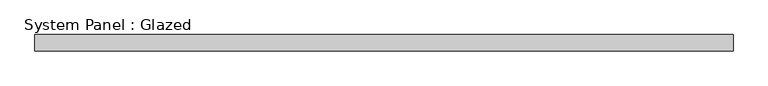
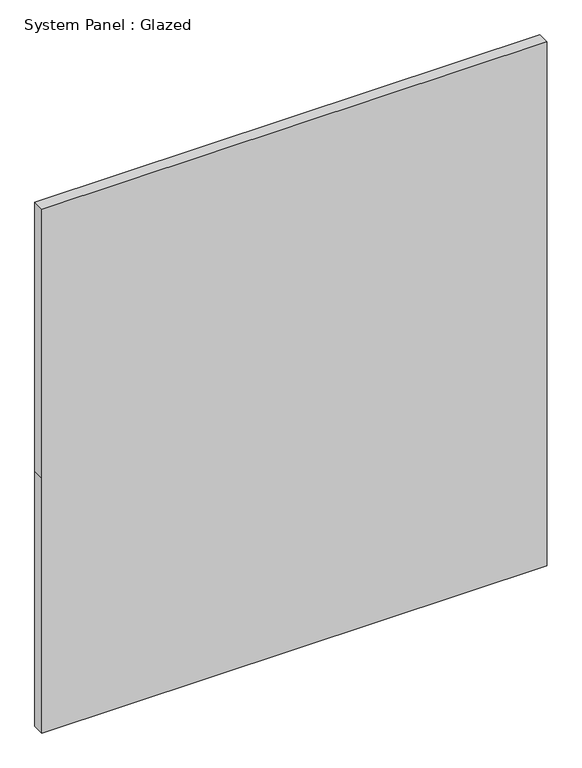
"""IFC4 building model written with IfcOpenShell, lengths in millimetres: plate geometry, System Panel : Glazed."""

import ifcopenshell
import ifcopenshell.guid

model = None  # the IFC model being written
_history = None  # IfcOwnerHistory: only IFC2X3 demands one
_inside = {}  # id of a spatial element -> (the spatial element, [elements in it])
_under = {}  # id of a project, library or spatial element -> (it, [spatial elements below it])
_declared = {}  # id of a project -> (the project, [libraries it declares])
_typed = {}  # id of a type object -> (the type object, [elements of that type])
_made_of = {}  # id of a material, layer set ... -> (it, [elements and type objects made of it])


def new_model(schema):
    """Start an empty IFC model of exactly this schema.

    Asked for "IFC4X3", IfcOpenShell would pick the latest addendum, in which some entities
    have other attributes; the version numbers below select the first issue.
    IFC2X3 requires an IfcOwnerHistory on every rooted entity: one is made here for all.
    """
    global model, _history
    if schema == "IFC4X3":
        model = ifcopenshell.file(schema_version=(4, 3, 0, 0))
    else:
        model = ifcopenshell.file(schema=schema)
    _inside.clear()
    _under.clear()
    _declared.clear()
    _typed.clear()
    _made_of.clear()
    _history = None
    if model.schema == "IFC2X3":
        org = make("IfcOrganization", Name="unknown")
        user = make(
            "IfcPersonAndOrganization",
            ThePerson=make("IfcPerson", FamilyName="unknown"),
            TheOrganization=org,
        )
        app = make(
            "IfcApplication",
            ApplicationDeveloper=org,
            Version="unknown",
            ApplicationFullName="unknown",
            ApplicationIdentifier="unknown",
        )
        _history = make(
            "IfcOwnerHistory",
            OwningUser=user,
            OwningApplication=app,
            ChangeAction="ADDED",
            CreationDate=0,
        )
    return model


def make(cls, **values):
    """One entity of the class cls with the attributes given. An attribute that is None is left unset."""
    return model.create_entity(
        cls, **{name: value for name, value in values.items() if value is not None}
    )


def rooted(cls, **values):
    """An entity with a GlobalId (a new one), such as an element, a storey or a relation."""
    return make(cls, GlobalId=ifcopenshell.guid.new(), OwnerHistory=_history, **values)


def si_unit(unit_type, name, prefix=None):
    """IfcSIUnit, for example si_unit("LENGTHUNIT", "METRE", prefix="MILLI")."""
    return make("IfcSIUnit", UnitType=unit_type, Prefix=prefix, Name=name)


def assignment(units):
    """IfcUnitAssignment: the units of a project."""
    return None if units is None else make("IfcUnitAssignment", Units=units)


def point(xyz):
    """IfcCartesianPoint."""
    return None if xyz is None else make("IfcCartesianPoint", Coordinates=xyz)


def direction(xyz):
    """IfcDirection."""
    return None if xyz is None else make("IfcDirection", DirectionRatios=xyz)


def frame(location, z_axis=None, x_axis=None):
    """IfcAxis2Placement3D, a coordinate frame: its origin and axes. An axis left out is left unset."""
    return make(
        "IfcAxis2Placement3D",
        Location=point(location),
        Axis=direction(z_axis),
        RefDirection=direction(x_axis),
    )


def origin():
    """The frame at (0, 0, 0) with its axes left unset."""
    return frame((0.0, 0.0, 0.0))


def place(relative_to, where):
    """IfcLocalPlacement: puts the frame where relative to a parent placement (None: the world)."""
    return make(
        "IfcLocalPlacement", PlacementRelTo=relative_to, RelativePlacement=where
    )


def context(
    kind, dimensions, precision=None, world=None, true_north=None, identifier=None
):
    """IfcGeometricRepresentationContext, for example the 3D "Model" context."""
    return make(
        "IfcGeometricRepresentationContext",
        ContextIdentifier=identifier,
        ContextType=kind,
        CoordinateSpaceDimension=dimensions,
        Precision=precision,
        WorldCoordinateSystem=world,
        TrueNorth=true_north,
    )


def project(units=None, contexts=None):
    """IfcProject with its units and contexts."""
    return rooted(
        "IfcProject",
        Name="project",
        RepresentationContexts=contexts,
        UnitsInContext=assignment(units),
    )


def spatial(cls, under=None, at=None, **own):
    """A site, building, storey or space (cls), placed at a placement, below another one or the project."""
    s = rooted(cls, ObjectPlacement=at, **own)
    if under is not None:
        _under.setdefault(under.id(), (under, []))[1].append(s)
    return s


def polyline(points):
    """IfcPolyline through the points."""
    return make("IfcPolyline", Points=[point(p) for p in points])


def outline(outer, holes=None, kind="AREA"):
    """IfcArbitraryClosedProfileDef: a profile drawn as a closed curve; with holes, ...WithVoids."""
    if holes is None:
        return make("IfcArbitraryClosedProfileDef", ProfileType=kind, OuterCurve=outer)
    return make(
        "IfcArbitraryProfileDefWithVoids",
        ProfileType=kind,
        OuterCurve=outer,
        InnerCurves=holes,
    )


def extrude(swept, where, along, depth):
    """IfcExtrudedAreaSolid: the profile swept, set in the frame where, extruded along a direction by depth."""
    return make(
        "IfcExtrudedAreaSolid",
        SweptArea=swept,
        Position=where,
        ExtrudedDirection=direction(along),
        Depth=depth,
    )


def shape(context_of_items, identifier, shape_type, items):
    """IfcShapeRepresentation: the items that make up one representation, for example the "Body"."""
    return make(
        "IfcShapeRepresentation",
        ContextOfItems=context_of_items,
        RepresentationIdentifier=identifier,
        RepresentationType=shape_type,
        Items=items,
    )


def source(mapping_origin, context_of_items, identifier, shape_type, items):
    """IfcRepresentationMap: a shape defined once, which mapped items show again and again."""
    return make(
        "IfcRepresentationMap",
        MappingOrigin=mapping_origin,
        MappedRepresentation=shape(context_of_items, identifier, shape_type, items),
    )


def transform(
    local_origin,
    x_axis=None,
    y_axis=None,
    z_axis=None,
    scale=None,
    scale2=None,
    scale3=None,
    uniform=True,
):
    """IfcCartesianTransformationOperator3D, or its non-uniform kind. x_axis, y_axis, z_axis: its Axis1, 2, 3."""
    if uniform:
        return make(
            "IfcCartesianTransformationOperator3D",
            Axis1=direction(x_axis),
            Axis2=direction(y_axis),
            LocalOrigin=point(local_origin),
            Scale=scale,
            Axis3=direction(z_axis),
        )
    return make(
        "IfcCartesianTransformationOperator3DnonUniform",
        Axis1=direction(x_axis),
        Axis2=direction(y_axis),
        LocalOrigin=point(local_origin),
        Scale=scale,
        Axis3=direction(z_axis),
        Scale2=scale2,
        Scale3=scale3,
    )


def mapped(mapping_source, mapping_target):
    """IfcMappedItem: shows the shape of a source again, moved by a transform."""
    return make(
        "IfcMappedItem", MappingSource=mapping_source, MappingTarget=mapping_target
    )


def made_of(thing, what):
    """Note that an element or type object is made of a material, layer set ...; save() writes the relation."""
    if what is not None:
        _made_of.setdefault(what.id(), (what, []))[1].append(thing)
    return thing


def element(
    cls,
    number,
    at=None,
    inside=None,
    cuts=None,
    type_object=None,
    material=None,
    context=None,
    identifier="Body",
    shape_type=None,
    held_by="IfcProductDefinitionShape",
    body=None,
    shapes=None,
    **own,
):
    """One element of the class cls, such as IfcWall. Its Tag is "e" and its number.

    at: its placement. inside: the storey or other place that contains it. cuts: it is an
    opening in that element (IfcRelVoidsElement). A single representation is given by context,
    identifier, shape_type and body (its items); several are given by shapes. held_by: the class
    of the entity that holds the representations. save() writes the other relations.
    """
    e = rooted(cls, Tag="e%d" % number, ObjectPlacement=at, **own)
    if body is not None:
        shapes = [shape(context, identifier, shape_type, body)]
    if shapes is not None:
        e.Representation = make(held_by, Representations=shapes)
    if inside is not None:
        _inside.setdefault(inside.id(), (inside, []))[1].append(e)
    if cuts is not None:
        rooted(
            "IfcRelVoidsElement", RelatingBuildingElement=cuts, RelatedOpeningElement=e
        )
    if type_object is not None:
        _typed.setdefault(type_object.id(), (type_object, []))[1].append(e)
    return made_of(e, material)


def aggregate(whole, parts):
    """IfcRelAggregates: a whole, such as a stair, and the parts it consists of."""
    return rooted("IfcRelAggregates", RelatingObject=whole, RelatedObjects=parts)


def save(model, path):
    """Write the relations noted so far, then the file.

    IfcRelAggregates (storeys below a building ...), IfcRelContainedInSpatialStructure (elements
    in a storey), IfcRelDefinesByType, IfcRelAssociatesMaterial and IfcRelDeclares: one each for
    every whole, place, type object, material and project.
    """
    for whole, parts in _under.values():
        aggregate(whole, parts)
    for where, things in _inside.values():
        rooted(
            "IfcRelContainedInSpatialStructure",
            RelatedElements=things,
            RelatingStructure=where,
        )
    for kind, things in _typed.values():
        rooted("IfcRelDefinesByType", RelatedObjects=things, RelatingType=kind)
    for what, things in _made_of.values():
        rooted("IfcRelAssociatesMaterial", RelatedObjects=things, RelatingMaterial=what)
    for by, libraries in _declared.values():
        rooted("IfcRelDeclares", RelatingContext=by, RelatedDefinitions=libraries)
    model.write(path)


def system_panel_glazed_99a56496(model_context):
    return source(origin(), model_context, "Body", "SweptSolid", [
        extrude(outline(polyline([(0.0, -541.655), (0.0, 541.655), (577.85, 541.655), (1187.45, 541.655), (1187.45, -541.655), (577.85, -541.655), (0.0, -541.655)])), frame((0.0, -44.45, 0.0), z_axis=(0.0, 1.0, 0.0), x_axis=(0.0, 0.0, 1.0)), (0.0, 0.0, 1.0), 25.4),
    ])


if __name__ == "__main__":
    model = new_model("IFC4")
    model_context = context("Model", 3, world=origin())
    ifc_project = project(units=[si_unit("LENGTHUNIT", "METRE", prefix="MILLI")], contexts=[model_context])
    site = spatial("IfcSite", under=ifc_project)
    building = spatial("IfcBuilding", under=site)
    placement = place(None, origin())
    system_panel_glazed_shape = system_panel_glazed_99a56496(model_context)
    element("IfcPlate", 1, ObjectType="System Panel : Glazed", at=placement, inside=building, context=model_context, shape_type="MappedRepresentation", body=[
        mapped(system_panel_glazed_shape, transform((0.0, 0.0, 0.0), x_axis=(1.0, 0.0, 0.0), y_axis=(0.0, 1.0, 0.0), z_axis=(0.0, 0.0, 1.0))),
    ])
    save(model, "model.ifc")

# Revit data of these elements
# Element 1 (IfcPlate, "System Panel : Glazed")
#   Materials on its faces: "Glass"
# Materials
#   "Glass": class "Unassigned", colour RGB 0 0 255, transparency 0.75
